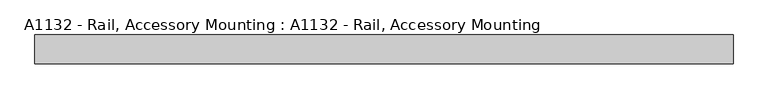
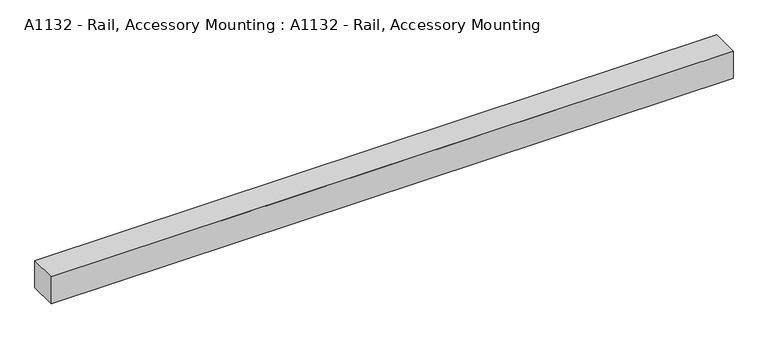
"""IFC4 building model written with IfcOpenShell, lengths in millimetres: proxy geometry, A1132 - Rail, Accessory Mounting : A1132 - Rail, Accessory Mounting."""

from ifc_helpers import new_model, si_unit, frame, origin, origin_with_axes, place, context, project, spatial, polyline, outline, extrude, source, transform, mapped, element, save


def a1132_rail_accessory_mounting_a1132_rail_accessory_mounting_24bb1397(model_context):
    return source(origin(), model_context, "Body", "SweptSolid", [
        extrude(outline(polyline([(609.6, -50.8), (-609.6, -50.8), (-609.6, 0.0), (609.6, 0.0), (609.6, -50.8)])), origin_with_axes(), (0.0, 0.0, 1.0), 50.8),
        extrude(outline(polyline([(-12.7, 25.4), (-12.7, 0.0), (-38.1, 0.0), (-38.1, 25.4), (-50.8, 25.4), (-50.8, 50.8), (0.0, 50.8), (0.0, 25.4), (-12.7, 25.4)])), frame((-304.8, 0.0, 0.0), z_axis=(1.0, 0.0, 0.0), x_axis=(0.0, 1.0, 0.0)), (0.0, 0.0, 1.0), 609.6),
    ])


if __name__ == "__main__":
    model = new_model("IFC4")
    model_context = context("Model", 3, world=origin())
    ifc_project = project(units=[si_unit("LENGTHUNIT", "METRE", prefix="MILLI")], contexts=[model_context])
    site = spatial("IfcSite", under=ifc_project)
    building = spatial("IfcBuilding", under=site)
    placement = place(None, origin())
    a1132_rail_accessory_mounting_a1132_rail_accessory_mounting_shape = a1132_rail_accessory_mounting_a1132_rail_accessory_mounting_24bb1397(model_context)
    element("IfcBuildingElementProxy", 1, Name="A1132 - Rail, Accessory Mounting : A1132 - Rail, Accessory Mounting", ObjectType="A1132 - Rail, Accessory Mounting : A1132 - Rail, Accessory Mounting", at=placement, inside=building, context=model_context, shape_type="MappedRepresentation", body=[
        mapped(a1132_rail_accessory_mounting_a1132_rail_accessory_mounting_shape, transform((0.0, 0.0, 0.0), x_axis=(1.0, 0.0, 0.0), y_axis=(0.0, 1.0, 0.0), z_axis=(0.0, 0.0, 1.0))),
    ])
    save(model, "model.ifc")

# Revit data of these elements
# Project information
#   Sheets - Total = "6"
#   Project Issue Date = "Issue Date"
#   Project Status = "Project Status"
#   Client Name = "Owner"
#   Project Address = "Enter address here"
#   Project Name = "Project Name"
#   Project Number = "Project Number"
#   Publication Date = "30-Jan-15"
# Type "A1132 - Rail, Accessory Mounting : A1132 - Rail, Accessory Mounting"
#   Watts2 = "0"
#   Watts1 = "0"
#   Unit_Issue = "LF"
#   UTIL_6_Misc = "-"
#   UTIL_5_NonMedGas = "-"
#   UTIL_4_MiscGas = "-"
#   UTIL_3_MedGas = "-"
#   UTIL_2_Elec = "-"
#   UTIL_1_WaterDrain = "-"
#   Nomenclature = "Rail, Accessory Mounting, 48\""
#   NSN = "6530"
#   Location [instance default] = ""
#   JSN = "A1132"
#   Fund_Source_VA = "-"
#   Fund_Source_Navy = "C"
#   Fund_Source_Army = "-"
#   Fund_Source_AF = "-"
#   ELEC_Volts2 = "0"
#   ELEC_Volts1 = "0"
#   ELEC_Phase2 = "0"
#   ELEC_Phase1 = "0"
#   ELEC_HertzSwitch = "0"
#   ELEC_HertzDependent = "0"
#   ELEC_Hertz = "0"
#   ELEC_Amps2 = "0"
#   ELEC_Amps1 = "0"
#   DetailDescription = "Horizontal mounting rail will consist of lock mounting devices capable of; supporting up to 75 pounds each, being repositioned, and mounting and dismounting of equipment without the use of tools. The rail must be capable of supporting medical equipment and accessories normally found in exam or patient rooms. The rail system must be capable of mounting and dismounting equipment without leaving or creating new holes in the finished surface of the wall."
#   CAT_VA = "A"
#   CAT_Navy = "A"
#   CAT_IHS = "-"
#   CAT_Army = "A"
#   CAT_AF = "A"
#   BTUperhour = "0"
#   Weight_IP = 5
#   Default Elevation = 4' - 0"
#   DIM_Width_IP = 4' - 0"
#   DIM_Height_IP = 0' - 2"
#   DIM_Depth_IP = 0' - 2"
#   CustomLength [instance default] = 4' - 0"
#   Assembly Code = ""
# Element 1 (IfcBuildingElementProxy, "A1132 - Rail, Accessory Mounting : A1132 - Rail, Accessory Mounting")
#   Location = "TREE1"
#   CustomLength = 2' - 0"
#   Materials on its faces: "EquipSpace"
# Materials
#   "EquipSpace": class "Miscellaneous", colour RGB 221 217 195, transparency 0.5
